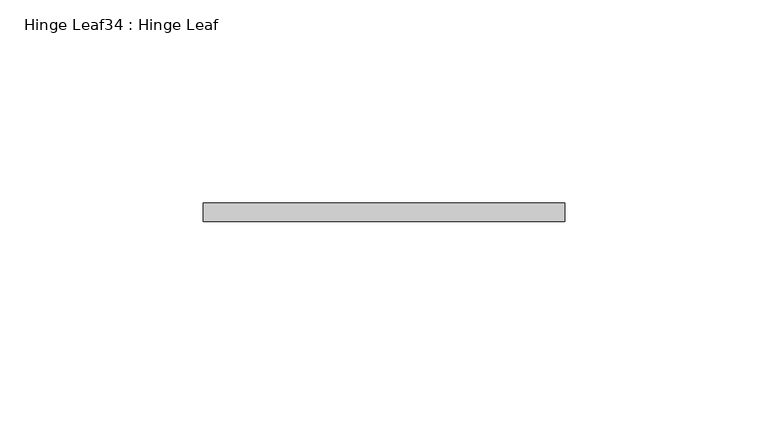
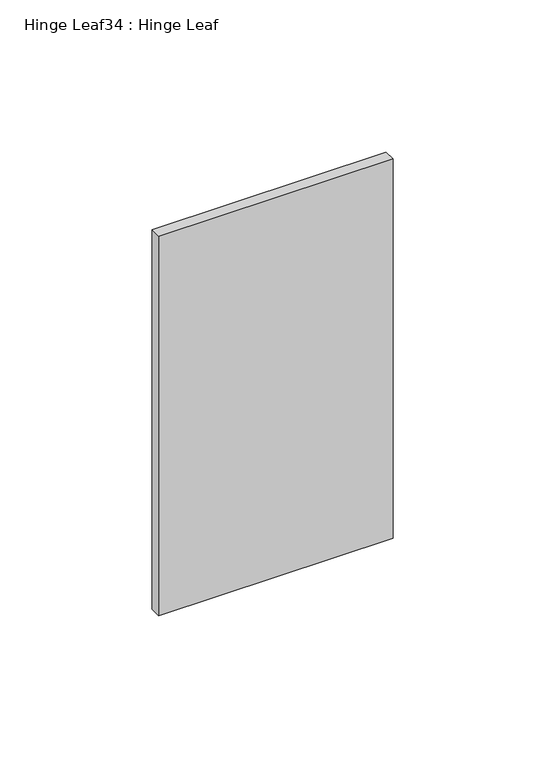
"""IFC4 building model written with IfcOpenShell, lengths in millimetres: proxy geometry, Hinge Leaf34 : Hinge Leaf."""

from ifc_helpers import new_model, si_unit, frame, origin, place, context, project, spatial, polyline, outline, extrude, source, transform, mapped, element, save


def hinge_leaf34_hinge_leaf_946f20d6(model_context):
    return source(origin(), model_context, "Body", "SweptSolid", [
        extrude(outline(polyline([(587327.7934739, -533980.5883841), (587327.7934739, -533976.0163841), (587416.6934739, -533976.0163841), (587416.6934739, -533980.5883841), (587327.7934739, -533980.5883841)])), frame((0.0, 0.0, 1936.75), z_axis=(0.0, 0.0, 1.0), x_axis=(1.0, 0.0, 0.0)), (0.0, 0.0, 1.0), 152.4),
    ])


if __name__ == "__main__":
    model = new_model("IFC4")
    model_context = context("Model", 3, world=origin())
    ifc_project = project(units=[si_unit("LENGTHUNIT", "METRE", prefix="MILLI")], contexts=[model_context])
    site = spatial("IfcSite", under=ifc_project)
    building = spatial("IfcBuilding", under=site)
    placement = place(None, origin())
    hinge_leaf34_hinge_leaf_shape = hinge_leaf34_hinge_leaf_946f20d6(model_context)
    element("IfcBuildingElementProxy", 1, Name="Hinge Leaf34 : Hinge Leaf", ObjectType="Hinge Leaf34 : Hinge Leaf", at=placement, inside=building, context=model_context, shape_type="MappedRepresentation", body=[
        mapped(hinge_leaf34_hinge_leaf_shape, transform((0.0, 0.0, 0.0), x_axis=(1.0, 0.0, 0.0), y_axis=(0.0, 1.0, 0.0), z_axis=(0.0, 0.0, 1.0))),
    ])
    save(model, "model.ifc")

# Revit data of these elements
# Element 1 (IfcBuildingElementProxy, "Hinge Leaf34 : Hinge Leaf")
#   Materials on its faces: "6\"X6\" WELD-ON STL BUTT HINGE"
# Materials
#   "6\"X6\" WELD-ON STL BUTT HINGE": class "Metal", colour RGB 189 187 185, transparency 0, Description = "Carbon steel", Cost = 0
